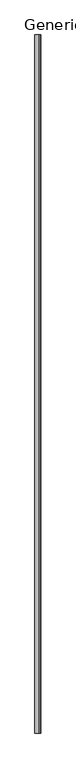
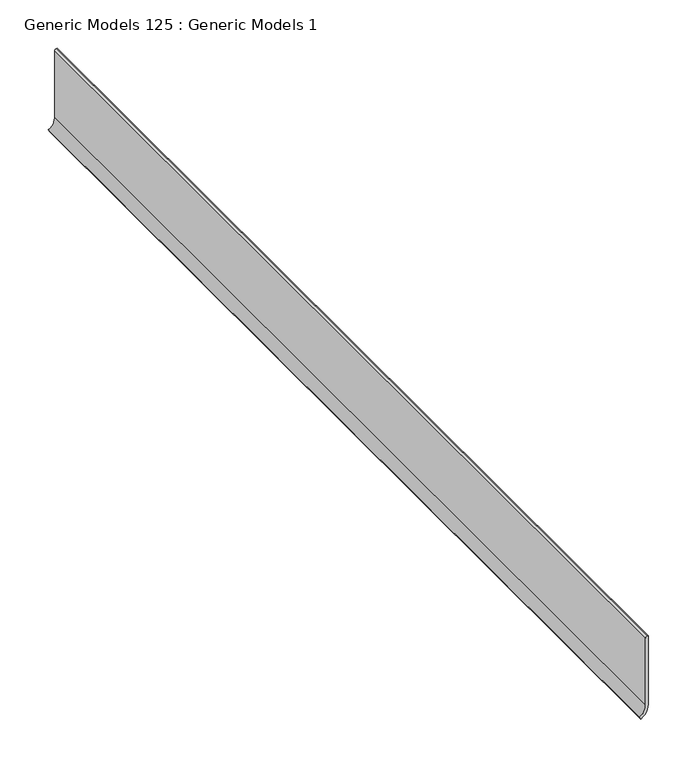
"""IFC4 building model written with IfcOpenShell, lengths in millimetres: proxy geometry, Generic Models 125 : Generic Models 1."""

from ifc_helpers import new_model, si_unit, point, frame, frame_2d, origin, place, context, project, spatial, polyline, circle_curve, trimmed, segment, composite_curve, outline, extrude, source, transform, mapped, element, save


def generic_models_125_generic_models_1_5b15c746(model_context):
    return source(origin(), model_context, "Body", "SweptSolid", [
        extrude(outline(composite_curve([segment(polyline([(-124.376067, 46827.9235531), (-124.376067, 46826.8353549)]), True, "CONTINUOUS"), segment(trimmed(circle_curve(frame_2d((-126.4628688, 46826.8353549)), 2.0868018), [point((-124.376067, 46826.8353549))], [point((-126.4628688, 46824.7485531))], False, "CARTESIAN"), True, "CONTINUOUS"), segment(polyline([(-126.4628688, 46824.7485531), (-210.5264363, 46824.7485531)]), True, "CONTINUOUS"), segment(trimmed(circle_curve(frame_2d((-210.5264363, 46810.0838562)), 14.6646968), [point((-210.5264363, 46824.7485531))], [point((-223.2264363, 46817.4162046))], True, "CARTESIAN"), True, "CONTINUOUS"), segment(polyline([(-223.2264363, 46817.4162046), (-225.976067, 46819.0037046)]), True, "CONTINUOUS"), segment(trimmed(circle_curve(frame_2d((-210.5264363, 46810.0838562)), 17.8396968), [point((-225.976067, 46819.0037046))], [point((-210.5264363, 46827.9235531))], False, "CARTESIAN"), True, "CONTINUOUS"), segment(polyline([(-210.5264363, 46827.9235531), (-124.376067, 46827.9235531)]), True, "CONTINUOUS")], self_intersect=False)), frame((0.0, 0.0, 0.0), z_axis=(0.0, 1.0, 0.0), x_axis=(0.0, 0.0, 1.0)), (0.0, 0.0, 1.0), 1219.2),
    ])


if __name__ == "__main__":
    model = new_model("IFC4")
    model_context = context("Model", 3, world=origin())
    ifc_project = project(units=[si_unit("LENGTHUNIT", "METRE", prefix="MILLI")], contexts=[model_context])
    site = spatial("IfcSite", under=ifc_project)
    building = spatial("IfcBuilding", under=site)
    placement = place(None, origin())
    generic_models_125_generic_models_1_shape = generic_models_125_generic_models_1_5b15c746(model_context)
    element("IfcBuildingElementProxy", 1, Name="Generic Models 125 : Generic Models 1", ObjectType="Generic Models 125 : Generic Models 1", at=placement, inside=building, context=model_context, shape_type="MappedRepresentation", body=[
        mapped(generic_models_125_generic_models_1_shape, transform((0.0, 0.0, 0.0), x_axis=(1.0, 0.0, 0.0), y_axis=(0.0, 1.0, 0.0), z_axis=(0.0, 0.0, 1.0))),
    ])
    save(model, "model.ifc")

# Revit data of these elements
# Element 1 (IfcBuildingElementProxy, "Generic Models 125 : Generic Models 1")
#   Materials on its faces: "MATCH EXISTING BASE"
# Materials
#   "MATCH EXISTING BASE": class "Generic", colour RGB 120 120 120, transparency 0, Cost = 0
